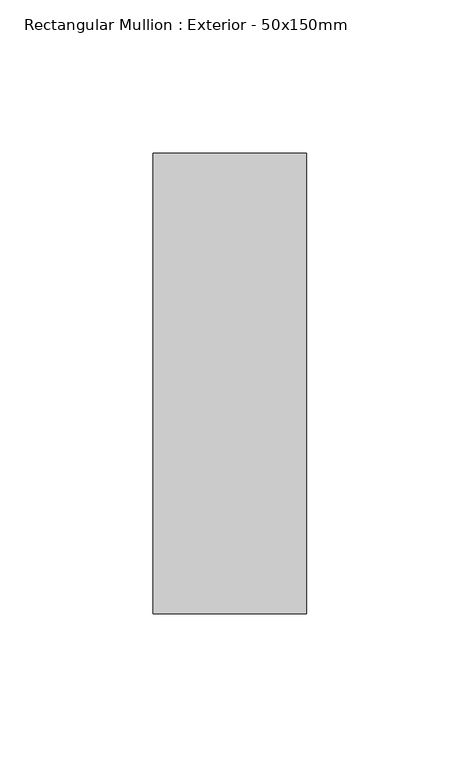
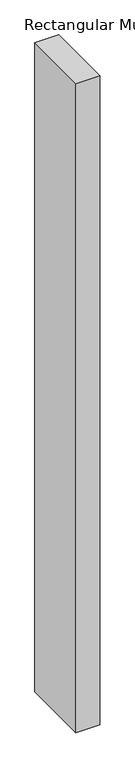
"""IFC4 building model written with IfcOpenShell, lengths in millimetres: member geometry, Rectangular Mullion : Exterior - 50x150mm."""

import ifcopenshell
import ifcopenshell.guid

model = None  # the IFC model being written
_history = None  # IfcOwnerHistory: only IFC2X3 demands one
_inside = {}  # id of a spatial element -> (the spatial element, [elements in it])
_under = {}  # id of a project, library or spatial element -> (it, [spatial elements below it])
_declared = {}  # id of a project -> (the project, [libraries it declares])
_typed = {}  # id of a type object -> (the type object, [elements of that type])
_made_of = {}  # id of a material, layer set ... -> (it, [elements and type objects made of it])


def new_model(schema):
    """Start an empty IFC model of exactly this schema.

    Asked for "IFC4X3", IfcOpenShell would pick the latest addendum, in which some entities
    have other attributes; the version numbers below select the first issue.
    IFC2X3 requires an IfcOwnerHistory on every rooted entity: one is made here for all.
    """
    global model, _history
    if schema == "IFC4X3":
        model = ifcopenshell.file(schema_version=(4, 3, 0, 0))
    else:
        model = ifcopenshell.file(schema=schema)
    _inside.clear()
    _under.clear()
    _declared.clear()
    _typed.clear()
    _made_of.clear()
    _history = None
    if model.schema == "IFC2X3":
        org = make("IfcOrganization", Name="unknown")
        user = make(
            "IfcPersonAndOrganization",
            ThePerson=make("IfcPerson", FamilyName="unknown"),
            TheOrganization=org,
        )
        app = make(
            "IfcApplication",
            ApplicationDeveloper=org,
            Version="unknown",
            ApplicationFullName="unknown",
            ApplicationIdentifier="unknown",
        )
        _history = make(
            "IfcOwnerHistory",
            OwningUser=user,
            OwningApplication=app,
            ChangeAction="ADDED",
            CreationDate=0,
        )
    return model


def make(cls, **values):
    """One entity of the class cls with the attributes given. An attribute that is None is left unset."""
    return model.create_entity(
        cls, **{name: value for name, value in values.items() if value is not None}
    )


def rooted(cls, **values):
    """An entity with a GlobalId (a new one), such as an element, a storey or a relation."""
    return make(cls, GlobalId=ifcopenshell.guid.new(), OwnerHistory=_history, **values)


def si_unit(unit_type, name, prefix=None):
    """IfcSIUnit, for example si_unit("LENGTHUNIT", "METRE", prefix="MILLI")."""
    return make("IfcSIUnit", UnitType=unit_type, Prefix=prefix, Name=name)


def assignment(units):
    """IfcUnitAssignment: the units of a project."""
    return None if units is None else make("IfcUnitAssignment", Units=units)


def point(xyz):
    """IfcCartesianPoint."""
    return None if xyz is None else make("IfcCartesianPoint", Coordinates=xyz)


def direction(xyz):
    """IfcDirection."""
    return None if xyz is None else make("IfcDirection", DirectionRatios=xyz)


def frame(location, z_axis=None, x_axis=None):
    """IfcAxis2Placement3D, a coordinate frame: its origin and axes. An axis left out is left unset."""
    return make(
        "IfcAxis2Placement3D",
        Location=point(location),
        Axis=direction(z_axis),
        RefDirection=direction(x_axis),
    )


def origin():
    """The frame at (0, 0, 0) with its axes left unset."""
    return frame((0.0, 0.0, 0.0))


def place(relative_to, where):
    """IfcLocalPlacement: puts the frame where relative to a parent placement (None: the world)."""
    return make(
        "IfcLocalPlacement", PlacementRelTo=relative_to, RelativePlacement=where
    )


def context(
    kind, dimensions, precision=None, world=None, true_north=None, identifier=None
):
    """IfcGeometricRepresentationContext, for example the 3D "Model" context."""
    return make(
        "IfcGeometricRepresentationContext",
        ContextIdentifier=identifier,
        ContextType=kind,
        CoordinateSpaceDimension=dimensions,
        Precision=precision,
        WorldCoordinateSystem=world,
        TrueNorth=true_north,
    )


def project(units=None, contexts=None):
    """IfcProject with its units and contexts."""
    return rooted(
        "IfcProject",
        Name="project",
        RepresentationContexts=contexts,
        UnitsInContext=assignment(units),
    )


def spatial(cls, under=None, at=None, **own):
    """A site, building, storey or space (cls), placed at a placement, below another one or the project."""
    s = rooted(cls, ObjectPlacement=at, **own)
    if under is not None:
        _under.setdefault(under.id(), (under, []))[1].append(s)
    return s


def polyline(points):
    """IfcPolyline through the points."""
    return make("IfcPolyline", Points=[point(p) for p in points])


def outline(outer, holes=None, kind="AREA"):
    """IfcArbitraryClosedProfileDef: a profile drawn as a closed curve; with holes, ...WithVoids."""
    if holes is None:
        return make("IfcArbitraryClosedProfileDef", ProfileType=kind, OuterCurve=outer)
    return make(
        "IfcArbitraryProfileDefWithVoids",
        ProfileType=kind,
        OuterCurve=outer,
        InnerCurves=holes,
    )


def extrude(swept, where, along, depth):
    """IfcExtrudedAreaSolid: the profile swept, set in the frame where, extruded along a direction by depth."""
    return make(
        "IfcExtrudedAreaSolid",
        SweptArea=swept,
        Position=where,
        ExtrudedDirection=direction(along),
        Depth=depth,
    )


def shape(context_of_items, identifier, shape_type, items):
    """IfcShapeRepresentation: the items that make up one representation, for example the "Body"."""
    return make(
        "IfcShapeRepresentation",
        ContextOfItems=context_of_items,
        RepresentationIdentifier=identifier,
        RepresentationType=shape_type,
        Items=items,
    )


def source(mapping_origin, context_of_items, identifier, shape_type, items):
    """IfcRepresentationMap: a shape defined once, which mapped items show again and again."""
    return make(
        "IfcRepresentationMap",
        MappingOrigin=mapping_origin,
        MappedRepresentation=shape(context_of_items, identifier, shape_type, items),
    )


def transform(
    local_origin,
    x_axis=None,
    y_axis=None,
    z_axis=None,
    scale=None,
    scale2=None,
    scale3=None,
    uniform=True,
):
    """IfcCartesianTransformationOperator3D, or its non-uniform kind. x_axis, y_axis, z_axis: its Axis1, 2, 3."""
    if uniform:
        return make(
            "IfcCartesianTransformationOperator3D",
            Axis1=direction(x_axis),
            Axis2=direction(y_axis),
            LocalOrigin=point(local_origin),
            Scale=scale,
            Axis3=direction(z_axis),
        )
    return make(
        "IfcCartesianTransformationOperator3DnonUniform",
        Axis1=direction(x_axis),
        Axis2=direction(y_axis),
        LocalOrigin=point(local_origin),
        Scale=scale,
        Axis3=direction(z_axis),
        Scale2=scale2,
        Scale3=scale3,
    )


def mapped(mapping_source, mapping_target):
    """IfcMappedItem: shows the shape of a source again, moved by a transform."""
    return make(
        "IfcMappedItem", MappingSource=mapping_source, MappingTarget=mapping_target
    )


def made_of(thing, what):
    """Note that an element or type object is made of a material, layer set ...; save() writes the relation."""
    if what is not None:
        _made_of.setdefault(what.id(), (what, []))[1].append(thing)
    return thing


def element(
    cls,
    number,
    at=None,
    inside=None,
    cuts=None,
    type_object=None,
    material=None,
    context=None,
    identifier="Body",
    shape_type=None,
    held_by="IfcProductDefinitionShape",
    body=None,
    shapes=None,
    **own,
):
    """One element of the class cls, such as IfcWall. Its Tag is "e" and its number.

    at: its placement. inside: the storey or other place that contains it. cuts: it is an
    opening in that element (IfcRelVoidsElement). A single representation is given by context,
    identifier, shape_type and body (its items); several are given by shapes. held_by: the class
    of the entity that holds the representations. save() writes the other relations.
    """
    e = rooted(cls, Tag="e%d" % number, ObjectPlacement=at, **own)
    if body is not None:
        shapes = [shape(context, identifier, shape_type, body)]
    if shapes is not None:
        e.Representation = make(held_by, Representations=shapes)
    if inside is not None:
        _inside.setdefault(inside.id(), (inside, []))[1].append(e)
    if cuts is not None:
        rooted(
            "IfcRelVoidsElement", RelatingBuildingElement=cuts, RelatedOpeningElement=e
        )
    if type_object is not None:
        _typed.setdefault(type_object.id(), (type_object, []))[1].append(e)
    return made_of(e, material)


def aggregate(whole, parts):
    """IfcRelAggregates: a whole, such as a stair, and the parts it consists of."""
    return rooted("IfcRelAggregates", RelatingObject=whole, RelatedObjects=parts)


def save(model, path):
    """Write the relations noted so far, then the file.

    IfcRelAggregates (storeys below a building ...), IfcRelContainedInSpatialStructure (elements
    in a storey), IfcRelDefinesByType, IfcRelAssociatesMaterial and IfcRelDeclares: one each for
    every whole, place, type object, material and project.
    """
    for whole, parts in _under.values():
        aggregate(whole, parts)
    for where, things in _inside.values():
        rooted(
            "IfcRelContainedInSpatialStructure",
            RelatedElements=things,
            RelatingStructure=where,
        )
    for kind, things in _typed.values():
        rooted("IfcRelDefinesByType", RelatedObjects=things, RelatingType=kind)
    for what, things in _made_of.values():
        rooted("IfcRelAssociatesMaterial", RelatedObjects=things, RelatingMaterial=what)
    for by, libraries in _declared.values():
        rooted("IfcRelDeclares", RelatingContext=by, RelatedDefinitions=libraries)
    model.write(path)


def rectangular_mullion_exterior_50x150mm_99e7c456(model_context):
    return source(origin(), model_context, "Body", "SweptSolid", [
        extrude(outline(polyline([(25.0, 0.0), (25.0, -150.0), (-25.0, -150.0), (-25.0, 0.0), (25.0, 0.0)])), frame((0.0, 0.0, -1449.9999999), z_axis=(0.0, 0.0, 1.0), x_axis=(1.0, 0.0, 0.0)), (0.0, 0.0, 1.0), 1449.9999999),
    ])


if __name__ == "__main__":
    model = new_model("IFC4")
    model_context = context("Model", 3, world=origin())
    ifc_project = project(units=[si_unit("LENGTHUNIT", "METRE", prefix="MILLI")], contexts=[model_context])
    site = spatial("IfcSite", under=ifc_project)
    building = spatial("IfcBuilding", under=site)
    placement = place(None, origin())
    rectangular_mullion_exterior_50x150mm_shape = rectangular_mullion_exterior_50x150mm_99e7c456(model_context)
    element("IfcMember", 1, ObjectType="Rectangular Mullion : Exterior - 50x150mm", at=placement, inside=building, context=model_context, shape_type="MappedRepresentation", body=[
        mapped(rectangular_mullion_exterior_50x150mm_shape, transform((0.0, 0.0, 0.0), x_axis=(1.0, 0.0, 0.0), y_axis=(0.0, 1.0, 0.0), z_axis=(0.0, 0.0, 1.0))),
    ])
    save(model, "model.ifc")

# Revit data of these elements
# Type "Rectangular Mullion : Exterior - 50x150mm"
#   built-in parameter 1007351 = -0.246063 (stored number, unit not read)
#   built-in parameter 1007304 = 0.492126 (stored number, unit not read)
#   built-in parameter 1007301 = 0.082021 (stored number, unit not read)
#   built-in parameter 1007300 = 0.082021 (stored number, unit not read)
# Element 1 (IfcMember, "Rectangular Mullion : Exterior - 50x150mm")
#   Materials on its faces: "Default Frame/Mullion (Interior/Exterior)"
# Materials
#   "Default Frame/Mullion (Interior/Exterior)": class "Generic", colour RGB 205 205 205, transparency 0, Description = "Udefineret karm/ramme materiale", Cost = 0
